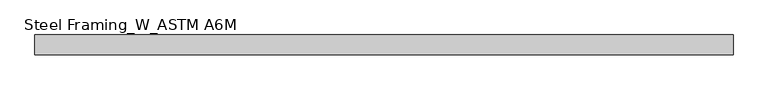
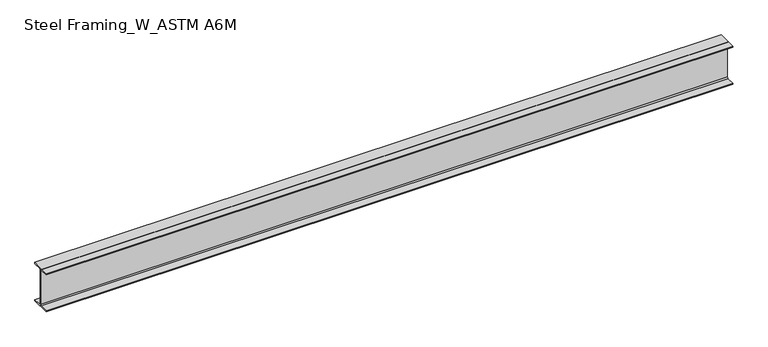
"""IFC4 building model written with IfcOpenShell, lengths in millimetres: beam geometry, Steel Framing_W_ASTM A6M : H_SB_AR_S02_W360x51_RG1."""

from ifc_helpers import new_model, si_unit, point, frame, frame_2d, origin, place, context, project, spatial, polyline, circle_curve, trimmed, segment, composite_curve, outline, extrude, source, transform, mapped, element, save


def steel_framing_w_astm_a6m_cdca116a(model_context):
    return source(origin(), model_context, "Body", "SweptSolid", [
        extrude(outline(composite_curve([segment(polyline([(85.5, -166.4), (85.5, -178.0), (-85.5, -178.0), (-85.5, -166.4), (-13.72, -166.4)]), True, "CONTINUOUS"), segment(trimmed(circle_curve(frame_2d((-13.72, -156.3)), 10.1), [point((-13.72, -166.4))], [point((-3.62, -156.3))], True, "CARTESIAN"), True, "CONTINUOUS"), segment(polyline([(-3.62, -156.3), (-3.62, 156.3)]), True, "CONTINUOUS"), segment(trimmed(circle_curve(frame_2d((-13.72, 156.3)), 10.1), [point((-3.62, 156.3))], [point((-13.72, 166.4))], True, "CARTESIAN"), True, "CONTINUOUS"), segment(polyline([(-13.72, 166.4), (-85.5, 166.4), (-85.5, 178.0), (85.5, 178.0), (85.5, 166.4), (13.72, 166.4)]), True, "CONTINUOUS"), segment(trimmed(circle_curve(frame_2d((13.72, 156.3)), 10.1), [point((13.72, 166.4))], [point((3.62, 156.3))], True, "CARTESIAN"), True, "CONTINUOUS"), segment(polyline([(3.62, 156.3), (3.62, -156.3)]), True, "CONTINUOUS"), segment(trimmed(circle_curve(frame_2d((13.72, -156.3)), 10.1), [point((3.62, -156.3))], [point((13.72, -166.4))], True, "CARTESIAN"), True, "CONTINUOUS"), segment(polyline([(13.72, -166.4), (85.5, -166.4)]), True, "CONTINUOUS")], self_intersect=False)), frame((-3014.9, 0.0, 0.0), z_axis=(1.0, 0.0, 0.0), x_axis=(0.0, 1.0, 0.0)), (0.0, 0.0, 1.0), 6029.8),
    ])


if __name__ == "__main__":
    model = new_model("IFC4")
    model_context = context("Model", 3, world=origin())
    ifc_project = project(units=[si_unit("LENGTHUNIT", "METRE", prefix="MILLI")], contexts=[model_context])
    site = spatial("IfcSite", under=ifc_project)
    building = spatial("IfcBuilding", under=site)
    placement = place(None, origin())
    steel_framing_w_astm_a6m_shape = steel_framing_w_astm_a6m_cdca116a(model_context)
    element("IfcBeam", 1, ObjectType="Steel Framing_W_ASTM A6M : H_SB_AR_S02_W360x51_RG1", at=placement, inside=building, context=model_context, shape_type="MappedRepresentation", body=[
        mapped(steel_framing_w_astm_a6m_shape, transform((0.0, 0.0, 0.0), x_axis=(1.0, 0.0, 0.0), y_axis=(0.0, 1.0, 0.0), z_axis=(0.0, 0.0, 1.0))),
    ])
    save(model, "model.ifc")

# Revit data of these elements
# Type "Steel Framing_W_ASTM A6M : H_SB_AR_S02_W360x51_RG1"
#   Type Mark = "RG1"
#   Section Name Key = "W14x34"
#   Width = 17.1 cm
#   Web Thickness = 0.724 cm
#   Web Fillet = 1.01 cm
#   Warping Constant = 287000.0 cm⁶
#   Torsional Moment of Inertia = 23.70 cm⁴
#   Section Area = 64.5 cm²
#   Plastic Modulus weak axis = 174.0 cm³
#   Plastic Modulus strong axis = 895.0 cm³
#   Perimeter = 1.36 m²/m
#   Nominal Weight = 51.00 kgf/m
#   Moment of Inertia weak axis = 970.00 cm⁴
#   Moment of Inertia strong axis = 14200.00 cm⁴
#   Height = 35.6 cm
#   Flange Thickness = 1.16 cm
#   Elastic Modulus weak axis = 113.0 cm³
#   Elastic Modulus strong axis = 796.0 cm³
#   Centroid Vertical = 17.8 cm
#   Centroid Horizontal = 8.55 cm
#   Length [instance default] = 1500 mm
#   Structural Material [instance default] = Steel, 45-345
#   Bolt Spacing = 0
#   Assembly Code = ""
# Element 1 (IfcBeam, "Steel Framing_W_ASTM A6M : H_SB_AR_S02_W360x51_RG1")
#   Materials on its faces: "Steel, 45-345"
# Materials
#   "Steel, 45-345": class "Metal", colour RGB 189 187 185, transparency 0, Description = "Steel 345 MPa", Cost = 0
